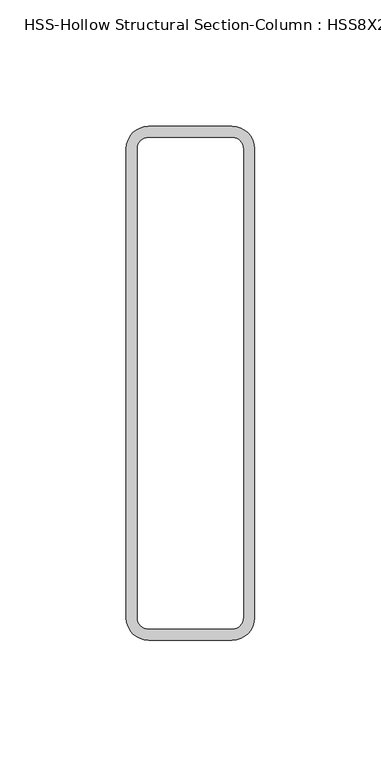
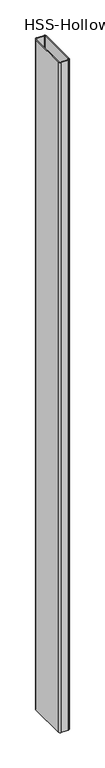
"""IFC4 building model written with IfcOpenShell, lengths in millimetres: column geometry, HSS-Hollow Structural Section-Column : HSS8X2X3/16."""

from ifc_helpers import new_model, si_unit, point, frame, frame_2d, origin, place, context, project, spatial, polyline, circle_curve, trimmed, segment, composite_curve, outline, extrude, source, transform, mapped, element, save


def hss_hollow_structural_section_column_hss8x2x3_16_588c78fd(model_context):
    return source(origin(), model_context, "Body", "SweptSolid", [
        extrude(outline(composite_curve([segment(trimmed(circle_curve(frame_2d((16.5608, 92.7608)), 8.8392), [point((16.5608, 101.6))], [point((25.4, 92.7608))], False, "CARTESIAN"), True, "CONTINUOUS"), segment(polyline([(25.4, 92.7608), (25.4, -92.7608)]), True, "CONTINUOUS"), segment(trimmed(circle_curve(frame_2d((16.5608, -92.7608)), 8.8392), [point((25.4, -92.7608))], [point((16.5608, -101.6))], False, "CARTESIAN"), True, "CONTINUOUS"), segment(polyline([(16.5608, -101.6), (-16.5608, -101.6)]), True, "CONTINUOUS"), segment(trimmed(circle_curve(frame_2d((-16.5608, -92.7608)), 8.8392), [point((-16.5608, -101.6))], [point((-25.4, -92.7608))], False, "CARTESIAN"), True, "CONTINUOUS"), segment(polyline([(-25.4, -92.7608), (-25.4, 92.7608)]), True, "CONTINUOUS"), segment(trimmed(circle_curve(frame_2d((-16.5608, 92.7608)), 8.8392), [point((-25.4, 92.7608))], [point((-16.5608, 101.6))], False, "CARTESIAN"), True, "CONTINUOUS"), segment(polyline([(-16.5608, 101.6), (16.5608, 101.6)]), True, "CONTINUOUS")], self_intersect=False), holes=[composite_curve([segment(polyline([(16.5608, 97.1804), (-16.5608, 97.1804)]), True, "CONTINUOUS"), segment(trimmed(circle_curve(frame_2d((-16.5608, 92.7608)), 4.4196), [point((-16.5608, 97.1804))], [point((-20.9804, 92.7608))], True, "CARTESIAN"), True, "CONTINUOUS"), segment(polyline([(-20.9804, 92.7608), (-20.9804, -92.7608)]), True, "CONTINUOUS"), segment(trimmed(circle_curve(frame_2d((-16.5608, -92.7608)), 4.4196), [point((-20.9804, -92.7608))], [point((-16.5608, -97.1804))], True, "CARTESIAN"), True, "CONTINUOUS"), segment(polyline([(-16.5608, -97.1804), (16.5608, -97.1804)]), True, "CONTINUOUS"), segment(trimmed(circle_curve(frame_2d((16.5608, -92.7608)), 4.4196), [point((16.5608, -97.1804))], [point((20.9804, -92.7608))], True, "CARTESIAN"), True, "CONTINUOUS"), segment(polyline([(20.9804, -92.7608), (20.9804, 92.7608)]), True, "CONTINUOUS"), segment(trimmed(circle_curve(frame_2d((16.5608, 92.7608)), 4.4196), [point((20.9804, 92.7608))], [point((16.5608, 97.1804))], True, "CARTESIAN"), True, "CONTINUOUS")], self_intersect=False)]), frame((0.0, 0.0, -350.0), z_axis=(0.0, 0.0, 1.0), x_axis=(1.0, 0.0, 0.0)), (0.0, 0.0, 1.0), 3350.0),
    ])


if __name__ == "__main__":
    model = new_model("IFC4")
    model_context = context("Model", 3, world=origin())
    ifc_project = project(units=[si_unit("LENGTHUNIT", "METRE", prefix="MILLI")], contexts=[model_context])
    site = spatial("IfcSite", under=ifc_project)
    building = spatial("IfcBuilding", under=site)
    placement = place(None, origin())
    hss_hollow_structural_section_column_hss8x2x3_16_shape = hss_hollow_structural_section_column_hss8x2x3_16_588c78fd(model_context)
    element("IfcColumn", 1, ObjectType="HSS-Hollow Structural Section-Column : HSS8X2X3/16", at=placement, inside=building, context=model_context, shape_type="MappedRepresentation", body=[
        mapped(hss_hollow_structural_section_column_hss8x2x3_16_shape, transform((0.0, 0.0, 0.0), x_axis=(1.0, 0.0, 0.0), y_axis=(0.0, 1.0, 0.0), z_axis=(0.0, 0.0, 1.0))),
    ])
    save(model, "model.ifc")

# Revit data of these elements
# Type "HSS-Hollow Structural Section-Column : HSS8X2X3/16"
#   Assembly Code = "B10"
#   Shape = "Rect."
#   Cost = 1
#   W = 12
#   Ht = 203.2 mm
#   b = 50.8 mm
#   kr = 8.839 mm
#   t = 4.42 mm
#   A = 0.00211612 m²
#   Structural Material [instance default] = Steel ASTM A500, Grade B, Rectangular and Square
# Element 1 (IfcColumn, "HSS-Hollow Structural Section-Column : HSS8X2X3/16")
#   Structural Material = Metal - Steel 43-275
#   Materials on its faces: "Metal - Steel 43-275"
# Materials
#   "Steel ASTM A500, Grade B, Rectangular and Square": class "Metal", colour RGB 199 199 199, transparency 0, Description = "Carbon steel", Cost = 0
#   "Metal - Steel 43-275": class "Metal", colour RGB 247 247 247, transparency 0, Cost = 0
